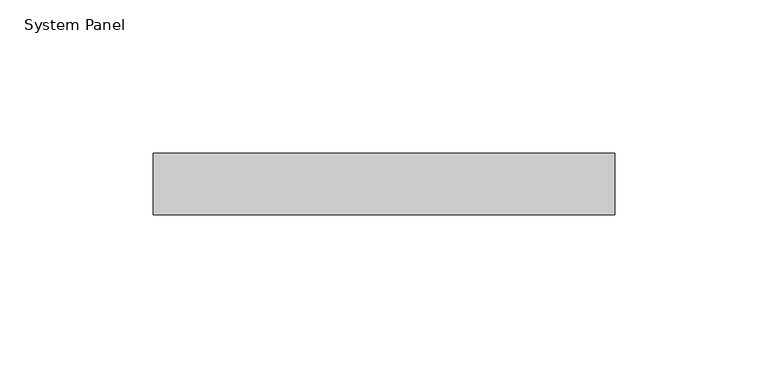
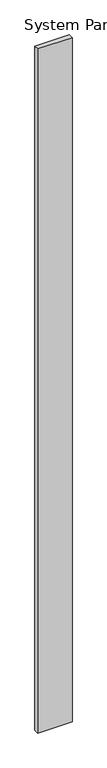
"""IFC4 building model written with IfcOpenShell, lengths in millimetres: plate geometry, System Panel : WWm-Glass-20mm-10mmOffset."""

from ifc_helpers import new_model, si_unit, origin, origin_with_axes, place, context, project, spatial, polyline, outline, extrude, source, transform, mapped, element, save


def system_panel_47d2be06(model_context):
    return source(origin(), model_context, "Body", "SweptSolid", [
        extrude(outline(polyline([(75.190733, 0.0), (-75.190733, 0.0), (-75.190733, 20.0), (75.190733, 20.0), (75.190733, 0.0)])), origin_with_axes(), (0.0, 0.0, 1.0), 3150.0),
    ])


if __name__ == "__main__":
    model = new_model("IFC4")
    model_context = context("Model", 3, world=origin())
    ifc_project = project(units=[si_unit("LENGTHUNIT", "METRE", prefix="MILLI")], contexts=[model_context])
    site = spatial("IfcSite", under=ifc_project)
    building = spatial("IfcBuilding", under=site)
    placement = place(None, origin())
    system_panel_shape = system_panel_47d2be06(model_context)
    element("IfcPlate", 1, ObjectType="System Panel : WWm-Glass-20mm-10mmOffset", at=placement, inside=building, context=model_context, shape_type="MappedRepresentation", body=[
        mapped(system_panel_shape, transform((0.0, 0.0, 0.0), x_axis=(1.0, 0.0, 0.0), y_axis=(0.0, 1.0, 0.0), z_axis=(0.0, 0.0, 1.0))),
    ])
    save(model, "model.ifc")

# Revit data of these elements
# Type "System Panel : WWm-Glass-20mm-10mmOffset"
#   Finish = ""
# Element 1 (IfcPlate, "System Panel : WWm-Glass-20mm-10mmOffset")
#   Materials on its faces: "WW-EC-GL-Storefront"
# Materials
#   "WW-EC-GL-Storefront": class "Glass", colour RGB 236 240 239, transparency 0.85, Description = "Storefront Glass", Cost = 0
